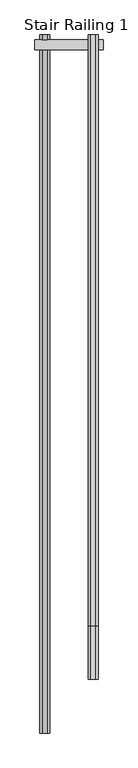
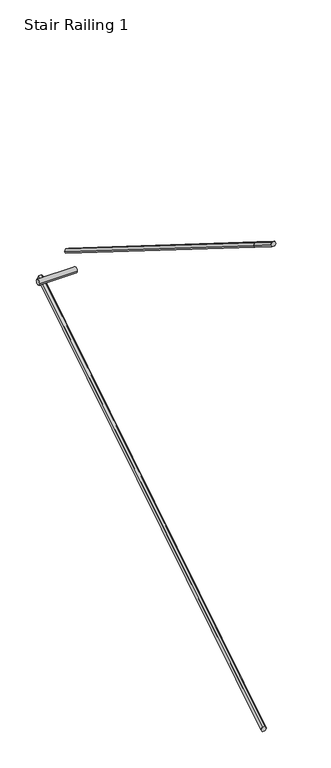
"""IFC4 building model written with IfcOpenShell, lengths in millimetres: railing geometry, Stair Railing 1."""

import ifcopenshell
import ifcopenshell.guid

model = None  # the IFC model being written
_history = None  # IfcOwnerHistory: only IFC2X3 demands one
_inside = {}  # id of a spatial element -> (the spatial element, [elements in it])
_under = {}  # id of a project, library or spatial element -> (it, [spatial elements below it])
_declared = {}  # id of a project -> (the project, [libraries it declares])
_typed = {}  # id of a type object -> (the type object, [elements of that type])
_made_of = {}  # id of a material, layer set ... -> (it, [elements and type objects made of it])


def new_model(schema):
    """Start an empty IFC model of exactly this schema.

    Asked for "IFC4X3", IfcOpenShell would pick the latest addendum, in which some entities
    have other attributes; the version numbers below select the first issue.
    IFC2X3 requires an IfcOwnerHistory on every rooted entity: one is made here for all.
    """
    global model, _history
    if schema == "IFC4X3":
        model = ifcopenshell.file(schema_version=(4, 3, 0, 0))
    else:
        model = ifcopenshell.file(schema=schema)
    _inside.clear()
    _under.clear()
    _declared.clear()
    _typed.clear()
    _made_of.clear()
    _history = None
    if model.schema == "IFC2X3":
        org = make("IfcOrganization", Name="unknown")
        user = make(
            "IfcPersonAndOrganization",
            ThePerson=make("IfcPerson", FamilyName="unknown"),
            TheOrganization=org,
        )
        app = make(
            "IfcApplication",
            ApplicationDeveloper=org,
            Version="unknown",
            ApplicationFullName="unknown",
            ApplicationIdentifier="unknown",
        )
        _history = make(
            "IfcOwnerHistory",
            OwningUser=user,
            OwningApplication=app,
            ChangeAction="ADDED",
            CreationDate=0,
        )
    return model


def make(cls, **values):
    """One entity of the class cls with the attributes given. An attribute that is None is left unset."""
    return model.create_entity(
        cls, **{name: value for name, value in values.items() if value is not None}
    )


def rooted(cls, **values):
    """An entity with a GlobalId (a new one), such as an element, a storey or a relation."""
    return make(cls, GlobalId=ifcopenshell.guid.new(), OwnerHistory=_history, **values)


def si_unit(unit_type, name, prefix=None):
    """IfcSIUnit, for example si_unit("LENGTHUNIT", "METRE", prefix="MILLI")."""
    return make("IfcSIUnit", UnitType=unit_type, Prefix=prefix, Name=name)


def assignment(units):
    """IfcUnitAssignment: the units of a project."""
    return None if units is None else make("IfcUnitAssignment", Units=units)


def point(xyz):
    """IfcCartesianPoint."""
    return None if xyz is None else make("IfcCartesianPoint", Coordinates=xyz)


def direction(xyz):
    """IfcDirection."""
    return None if xyz is None else make("IfcDirection", DirectionRatios=xyz)


def frame(location, z_axis=None, x_axis=None):
    """IfcAxis2Placement3D, a coordinate frame: its origin and axes. An axis left out is left unset."""
    return make(
        "IfcAxis2Placement3D",
        Location=point(location),
        Axis=direction(z_axis),
        RefDirection=direction(x_axis),
    )


def origin():
    """The frame at (0, 0, 0) with its axes left unset."""
    return frame((0.0, 0.0, 0.0))


def place(relative_to, where):
    """IfcLocalPlacement: puts the frame where relative to a parent placement (None: the world)."""
    return make(
        "IfcLocalPlacement", PlacementRelTo=relative_to, RelativePlacement=where
    )


def context(
    kind, dimensions, precision=None, world=None, true_north=None, identifier=None
):
    """IfcGeometricRepresentationContext, for example the 3D "Model" context."""
    return make(
        "IfcGeometricRepresentationContext",
        ContextIdentifier=identifier,
        ContextType=kind,
        CoordinateSpaceDimension=dimensions,
        Precision=precision,
        WorldCoordinateSystem=world,
        TrueNorth=true_north,
    )


def project(units=None, contexts=None):
    """IfcProject with its units and contexts."""
    return rooted(
        "IfcProject",
        Name="project",
        RepresentationContexts=contexts,
        UnitsInContext=assignment(units),
    )


def spatial(cls, under=None, at=None, **own):
    """A site, building, storey or space (cls), placed at a placement, below another one or the project."""
    s = rooted(cls, ObjectPlacement=at, **own)
    if under is not None:
        _under.setdefault(under.id(), (under, []))[1].append(s)
    return s


def circle_curve(where, radius):
    """IfcCircle in the frame where."""
    return make("IfcCircle", Position=where, Radius=radius)


def faces_of(points, faces, orient=None, outer=None):
    """IfcFace entities. A face is a list of loops; a loop is a list of indices into points, from 0.

    orient and outer hold one flag for each loop. By default every Orientation is true, the
    first loop of a face is its IfcFaceOuterBound and the others are IfcFaceBound.
    """
    made = []
    for i, loops in enumerate(faces):
        bounds = []
        for j, loop in enumerate(loops):
            is_outer = j == 0 if outer is None else outer[i][j]
            bounds.append(
                make(
                    "IfcFaceOuterBound" if is_outer else "IfcFaceBound",
                    Bound=make("IfcPolyLoop", Polygon=[points[k] for k in loop]),
                    Orientation=True if orient is None else orient[i][j],
                )
            )
        made.append(make("IfcFace", Bounds=bounds))
    return made


def faceted_brep(points, faces, orient=None, outer=None, voids=None):
    """IfcFacetedBrep: a solid bounded by flat faces; with voids (closed shells), ...WithVoids."""
    shared = [point(p) for p in points]
    hull = make("IfcClosedShell", CfsFaces=faces_of(shared, faces, orient, outer))
    if voids is None:
        return make("IfcFacetedBrep", Outer=hull)
    return make(
        "IfcFacetedBrepWithVoids",
        Outer=hull,
        Voids=[
            make(cls, CfsFaces=faces_of(shared, fs, o, b)) for cls, fs, o, b in voids
        ],
    )


def shape(context_of_items, identifier, shape_type, items):
    """IfcShapeRepresentation: the items that make up one representation, for example the "Body"."""
    return make(
        "IfcShapeRepresentation",
        ContextOfItems=context_of_items,
        RepresentationIdentifier=identifier,
        RepresentationType=shape_type,
        Items=items,
    )


def source(mapping_origin, context_of_items, identifier, shape_type, items):
    """IfcRepresentationMap: a shape defined once, which mapped items show again and again."""
    return make(
        "IfcRepresentationMap",
        MappingOrigin=mapping_origin,
        MappedRepresentation=shape(context_of_items, identifier, shape_type, items),
    )


def transform(
    local_origin,
    x_axis=None,
    y_axis=None,
    z_axis=None,
    scale=None,
    scale2=None,
    scale3=None,
    uniform=True,
):
    """IfcCartesianTransformationOperator3D, or its non-uniform kind. x_axis, y_axis, z_axis: its Axis1, 2, 3."""
    if uniform:
        return make(
            "IfcCartesianTransformationOperator3D",
            Axis1=direction(x_axis),
            Axis2=direction(y_axis),
            LocalOrigin=point(local_origin),
            Scale=scale,
            Axis3=direction(z_axis),
        )
    return make(
        "IfcCartesianTransformationOperator3DnonUniform",
        Axis1=direction(x_axis),
        Axis2=direction(y_axis),
        LocalOrigin=point(local_origin),
        Scale=scale,
        Axis3=direction(z_axis),
        Scale2=scale2,
        Scale3=scale3,
    )


def mapped(mapping_source, mapping_target):
    """IfcMappedItem: shows the shape of a source again, moved by a transform."""
    return make(
        "IfcMappedItem", MappingSource=mapping_source, MappingTarget=mapping_target
    )


def made_of(thing, what):
    """Note that an element or type object is made of a material, layer set ...; save() writes the relation."""
    if what is not None:
        _made_of.setdefault(what.id(), (what, []))[1].append(thing)
    return thing


def element(
    cls,
    number,
    at=None,
    inside=None,
    cuts=None,
    type_object=None,
    material=None,
    context=None,
    identifier="Body",
    shape_type=None,
    held_by="IfcProductDefinitionShape",
    body=None,
    shapes=None,
    **own,
):
    """One element of the class cls, such as IfcWall. Its Tag is "e" and its number.

    at: its placement. inside: the storey or other place that contains it. cuts: it is an
    opening in that element (IfcRelVoidsElement). A single representation is given by context,
    identifier, shape_type and body (its items); several are given by shapes. held_by: the class
    of the entity that holds the representations. save() writes the other relations.
    """
    e = rooted(cls, Tag="e%d" % number, ObjectPlacement=at, **own)
    if body is not None:
        shapes = [shape(context, identifier, shape_type, body)]
    if shapes is not None:
        e.Representation = make(held_by, Representations=shapes)
    if inside is not None:
        _inside.setdefault(inside.id(), (inside, []))[1].append(e)
    if cuts is not None:
        rooted(
            "IfcRelVoidsElement", RelatingBuildingElement=cuts, RelatedOpeningElement=e
        )
    if type_object is not None:
        _typed.setdefault(type_object.id(), (type_object, []))[1].append(e)
    return made_of(e, material)


def aggregate(whole, parts):
    """IfcRelAggregates: a whole, such as a stair, and the parts it consists of."""
    return rooted("IfcRelAggregates", RelatingObject=whole, RelatedObjects=parts)


def save(model, path):
    """Write the relations noted so far, then the file.

    IfcRelAggregates (storeys below a building ...), IfcRelContainedInSpatialStructure (elements
    in a storey), IfcRelDefinesByType, IfcRelAssociatesMaterial and IfcRelDeclares: one each for
    every whole, place, type object, material and project.
    """
    for whole, parts in _under.values():
        aggregate(whole, parts)
    for where, things in _inside.values():
        rooted(
            "IfcRelContainedInSpatialStructure",
            RelatedElements=things,
            RelatingStructure=where,
        )
    for kind, things in _typed.values():
        rooted("IfcRelDefinesByType", RelatedObjects=things, RelatingType=kind)
    for what, things in _made_of.values():
        rooted("IfcRelAssociatesMaterial", RelatedObjects=things, RelatingMaterial=what)
    for by, libraries in _declared.values():
        rooted("IfcRelDeclares", RelatingContext=by, RelatedDefinitions=libraries)
    model.write(path)


def plane_surface(at):
    """IfcPlane: the flat surface through the origin of the frame at, square to its z axis."""
    return make("IfcPlane", Position=at)


def cylinder_surface(at, radius):
    """IfcCylindricalSurface: all points at the distance radius from the z axis of the frame at."""
    return make("IfcCylindricalSurface", Position=at, Radius=radius)


def advanced_brep(points, edges, surfaces, faces):
    """IfcAdvancedBrep: a solid bounded by faces that lie on surfaces and meet in shared edges.

    An edge is (start, end): straight between two places in points (the first is 0);
    or (start, end, curve); or (start, end, curve, False) where it runs against its curve.
    A face is (place in surfaces, loops), or (place, loops, False) where it looks against
    its surface's normal. A loop lists edges by number (the first is 1), with a minus sign
    where the edge is run from its end to its start. The first loop is the outer one.
    """
    corners = [point(p) for p in points]
    vertices = [make("IfcVertexPoint", VertexGeometry=c) for c in corners]
    made = []
    for start, end, *more in edges:
        made.append(
            make(
                "IfcEdgeCurve",
                EdgeStart=vertices[start],
                EdgeEnd=vertices[end],
                EdgeGeometry=more[0] if more else make("IfcPolyline", Points=[corners[start], corners[end]]),
                SameSense=more[1] if len(more) > 1 else True,
            )
        )
    hull = []
    for where, loops, *sense in faces:
        bounds = []
        for j, loop in enumerate(loops):
            ring = [make("IfcOrientedEdge", EdgeElement=made[abs(k) - 1], Orientation=k > 0) for k in loop]
            bounds.append(
                make(
                    "IfcFaceOuterBound" if j == 0 else "IfcFaceBound",
                    Bound=make("IfcEdgeLoop", EdgeList=ring),
                    Orientation=True,
                )
            )
        hull.append(make("IfcAdvancedFace", Bounds=bounds, FaceSurface=surfaces[where], SameSense=sense[0] if sense else True))
    return make("IfcAdvancedBrep", Outer=make("IfcClosedShell", CfsFaces=hull))


def stair_railing_1_d4a7e100(model_context):
    return source(origin(), model_context, "Body", "SolidModel", [
        faceted_brep([(-1415.3134126, 56357.2066802, 9028.2888889), (-1428.0134126, 56357.2066802, 9006.2918436), (-1453.4134126, 56357.2066802, 9006.2918436), (-1466.1134126, 56357.2066802, 9028.2888889), (-1453.4134126, 56357.2066802, 9050.2859341), (-1428.0134126, 56357.2066802, 9050.2859341), (-1415.3134126, 52725.0066802, 6753.5777778), (-1428.0134126, 52725.0066802, 6775.574823), (-1453.4134126, 52725.0066802, 6775.574823), (-1466.1134126, 52725.0066802, 6753.5777778), (-1453.4134126, 52725.0066802, 6731.5807325), (-1428.0134126, 52725.0066802, 6731.5807325)], [[[0, 1, 2, 3, 4, 5]], [[6, 7, 8, 9, 10, 11]], [[1, 0, 6, 11]], [[2, 1, 11, 10]], [[3, 2, 10, 9]], [[4, 3, 9, 8]], [[5, 4, 8, 7]], [[0, 5, 7, 6]]]),
        advanced_brep(
        [(-1136.9891104, 56281.0066802, 9028.2888889), (-1136.9891104, 56331.8066802, 9028.2888889), (-1491.5134126, 56281.0066802, 9028.2888889), (-1491.5134126, 56331.8066802, 9028.2888889)],
        [
            (0, 1, circle_curve(frame((-1136.9891104, 56306.4066802, 9028.2888889), z_axis=(1.0, 0.0, 0.0), x_axis=(0.0, -1.0, 0.0)), 25.4)),
            (1, 0, circle_curve(frame((-1136.9891104, 56306.4066802, 9028.2888889), z_axis=(1.0, 0.0, 0.0), x_axis=(0.0, -1.0, 0.0)), 25.4)),
            (2, 3, circle_curve(frame((-1491.5134126, 56306.4066802, 9028.2888889), z_axis=(-1.0, 0.0, 0.0), x_axis=(0.0, -1.0, 0.0)), 25.4)),
            (3, 2, circle_curve(frame((-1491.5134126, 56306.4066802, 9028.2888889), z_axis=(-1.0, 0.0, 0.0), x_axis=(0.0, -1.0, 0.0)), 25.4)),
            (0, 2),
            (3, 1),
        ],
        [
            plane_surface(frame((-1136.9891104, 56281.0066802, 9002.8888889), z_axis=(1.0, 0.0, 0.0), x_axis=(0.0, 1.0, 0.0))),
            plane_surface(frame((-1491.5134126, 56281.0066802, 9002.8888889), z_axis=(-1.0, 0.0, 0.0), x_axis=(0.0, -1.0, 0.0))),
            cylinder_surface(frame((-1491.5134126, 56306.4066802, 9028.2888889), z_axis=(1.0, 0.0, 0.0), x_axis=(0.0, -1.0, 0.0)), 25.4),
        ],
        [
            (0, [[1, 2]]),
            (1, [[3, 4]]),
            (2, [[-1, 5, -4, 6]]),
            (2, [[-2, -6, -3, -5]]),
        ],
    ),
        faceted_brep([(-1213.1891104, 53283.8066802, 11128.0222222), (-1200.4891104, 53283.8066802, 11106.025177), (-1175.0891104, 53283.8066802, 11106.025177), (-1162.3891104, 53283.8066802, 11128.0222222), (-1175.0891104, 53283.8066802, 11150.0192675), (-1200.4891104, 53283.8066802, 11150.0192675), (-1213.1891104, 56357.2066802, 9203.2666667), (-1200.4891104, 56357.2066802, 9225.2637119), (-1175.0891104, 56357.2066802, 9225.2637119), (-1162.3891104, 56357.2066802, 9203.2666667), (-1175.0891104, 56357.2066802, 9181.2696214), (-1200.4891104, 56357.2066802, 9181.2696214)], [[[0, 1, 2, 3, 4, 5]], [[6, 7, 8, 9, 10, 11]], [[1, 0, 6, 11]], [[2, 1, 11, 10]], [[3, 2, 10, 9]], [[4, 3, 9, 8]], [[5, 4, 8, 7]], [[0, 5, 7, 6]]]),
        faceted_brep([(-1213.1891104, 53004.4066802, 11303.0), (-1200.4891104, 53004.4066802, 11281.0029547), (-1175.0891104, 53004.4066802, 11281.0029547), (-1162.3891104, 53004.4066802, 11303.0), (-1175.0891104, 53004.4066802, 11324.9970453), (-1200.4891104, 53004.4066802, 11324.9970453), (-1213.1891104, 53283.8066802, 11128.0222222), (-1200.4891104, 53283.8066802, 11150.0192675), (-1175.0891104, 53283.8066802, 11150.0192675), (-1162.3891104, 53283.8066802, 11128.0222222), (-1175.0891104, 53283.8066802, 11106.025177), (-1200.4891104, 53283.8066802, 11106.025177)], [[[0, 1, 2, 3, 4, 5]], [[6, 7, 8, 9, 10, 11]], [[1, 0, 6, 11]], [[2, 1, 11, 10]], [[3, 2, 10, 9]], [[4, 3, 9, 8]], [[5, 4, 8, 7]], [[0, 5, 7, 6]]]),
    ])


if __name__ == "__main__":
    model = new_model("IFC4")
    model_context = context("Model", 3, world=origin())
    ifc_project = project(units=[si_unit("LENGTHUNIT", "METRE", prefix="MILLI")], contexts=[model_context])
    site = spatial("IfcSite", under=ifc_project)
    building = spatial("IfcBuilding", under=site)
    placement = place(None, origin())
    stair_railing_1_shape = stair_railing_1_d4a7e100(model_context)
    element("IfcRailing", 1, ObjectType="Stair Railing 1", at=placement, inside=building, context=model_context, shape_type="MappedRepresentation", body=[
        mapped(stair_railing_1_shape, transform((0.0, 0.0, 0.0), x_axis=(1.0, 0.0, 0.0), y_axis=(0.0, 1.0, 0.0), z_axis=(0.0, 0.0, 1.0))),
    ])
    save(model, "model.ifc")
